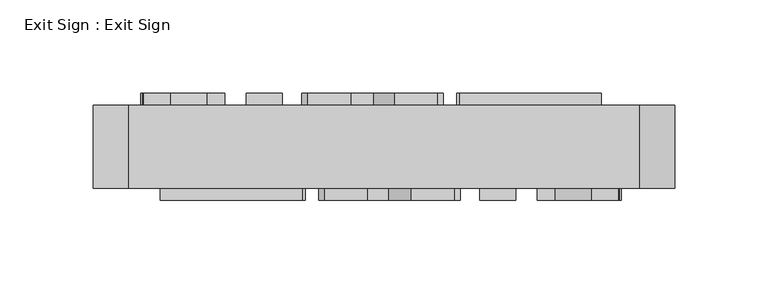
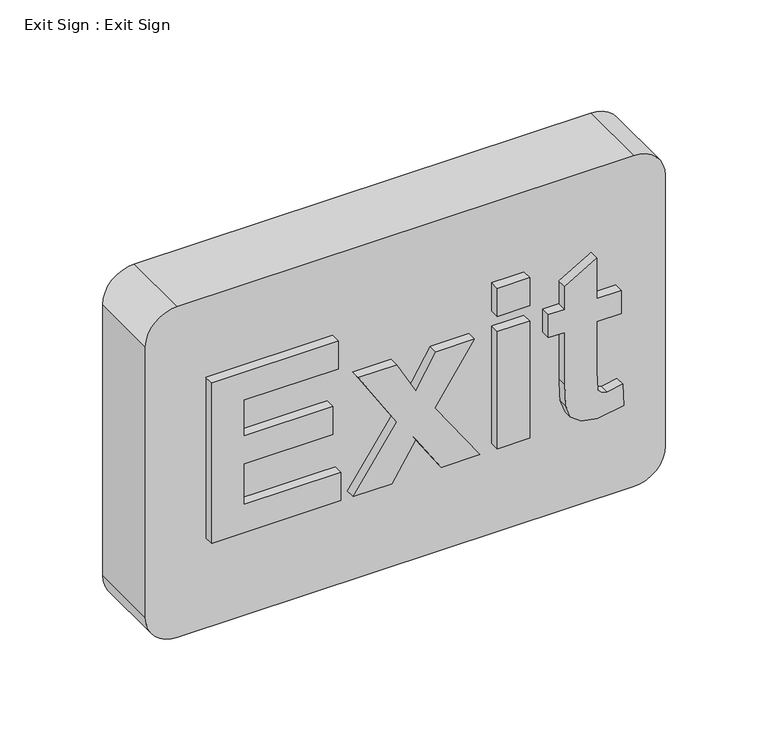
"""IFC4 building model written with IfcOpenShell, lengths in millimetres: proxy geometry, Exit Sign : Exit Sign."""

from ifc_helpers import new_model, si_unit, point, frame, frame_2d, origin, place, context, project, spatial, polyline, circle_curve, trimmed, segment, composite_curve, outline, extrude, source, transform, mapped, element, save


def exit_sign_exit_sign_daf696ad(model_context):
    return source(origin(), model_context, "Body", "SweptSolid", [
        extrude(outline(composite_curve([segment(polyline([(2438.4, 136.525), (2438.4, -136.525)]), True, "CONTINUOUS"), segment(trimmed(circle_curve(frame_2d((2419.35, -136.525)), 19.05), [point((2438.4, -136.525))], [point((2419.35, -155.575))], False, "CARTESIAN"), True, "CONTINUOUS"), segment(polyline([(2419.35, -155.575), (2247.9, -155.575)]), True, "CONTINUOUS"), segment(trimmed(circle_curve(frame_2d((2247.9, -136.525)), 19.05), [point((2247.9, -155.575))], [point((2228.85, -136.525))], False, "CARTESIAN"), True, "CONTINUOUS"), segment(polyline([(2228.85, -136.525), (2228.85, 136.525)]), True, "CONTINUOUS"), segment(trimmed(circle_curve(frame_2d((2247.9, 136.525)), 19.05), [point((2228.85, 136.525))], [point((2247.9, 155.575))], False, "CARTESIAN"), True, "CONTINUOUS"), segment(polyline([(2247.9, 155.575), (2419.35, 155.575)]), True, "CONTINUOUS"), segment(trimmed(circle_curve(frame_2d((2419.35, 136.525)), 19.05), [point((2419.35, 155.575))], [point((2438.4, 136.525))], False, "CARTESIAN"), True, "CONTINUOUS")], self_intersect=False)), frame((0.0, -34.925, 0.0), z_axis=(0.0, 1.0, 0.0), x_axis=(0.0, 0.0, 1.0)), (0.0, 0.0, 1.0), 44.45),
        extrude(outline(polyline([(2286.4280581, -119.6667099), (2286.4280581, -42.2571861), (2304.1677406, -42.2571861), (2304.1677406, -100.314329), (2329.9709152, -100.314329), (2329.9709152, -47.0952813), (2347.7105977, -47.0952813), (2347.7105977, -100.314329), (2370.2883755, -100.314329), (2370.2883755, -43.8698845), (2388.0280581, -43.8698845), (2388.0280581, -119.6667099), (2286.4280581, -119.6667099)])), frame((0.0, -41.275, 0.0), z_axis=(0.0, 1.0, 0.0), x_axis=(0.0, 0.0, 1.0)), (0.0, 0.0, 1.0), 6.35),
        extrude(outline(polyline([(2286.4280581, -35.0000432), (2286.4280581, -11.9938925), (2309.4090104, 2.4195996), (2286.4280581, 17.7906314), (2286.4280581, 40.7967822), (2325.4855977, 13.9100758), (2360.612185, 37.5713853), (2360.612185, 14.5652345), (2340.2266692, 2.4195996), (2360.612185, -8.7684956), (2360.612185, -31.7746464), (2324.6288517, -8.793694), (2286.4280581, -35.0000432)])), frame((0.0, -41.275, 0.0), z_axis=(0.0, 1.0, 0.0), x_axis=(0.0, 0.0, 1.0)), (0.0, 0.0, 1.0), 6.35),
        extrude(outline(polyline([(70.6317028, -41.275), (51.2793218, -41.275), (51.2793218, -34.925), (70.6317028, -34.925), (70.6317028, -41.275)])), frame((0.0, 0.0, 2370.2883755), z_axis=(0.0, 0.0, 1.0), x_axis=(1.0, 0.0, 0.0)), (0.0, 0.0, 1.0), 17.7396825),
        extrude(outline(polyline([(70.6317028, -41.275), (51.2793218, -41.275), (51.2793218, -34.925), (70.6317028, -34.925), (70.6317028, -41.275)])), frame((0.0, 0.0, 2286.4280581), z_axis=(0.0, 0.0, 1.0), x_axis=(1.0, 0.0, 0.0)), (0.0, 0.0, 1.0), 74.184127),
        extrude(outline(polyline([(2360.612185, 125.4634488), (2360.612185, 110.9491631), (2386.4153597, 110.9491631), (2375.1264708, 91.5967822), (2360.612185, 91.5967822), (2360.612185, 81.9205917), (2346.0978993, 81.9205917), (2346.0978993, 91.5967822), (2313.1887723, 91.5967822), (2299.1028597, 92.2267425), (2291.3165501, 95.0615639), (2286.6296454, 101.4493615), (2284.8153597, 111.2263456), (2287.4359946, 127.0761472), (2301.1943279, 126.269798), (2299.3296454, 117.1983695), (2300.3753795, 113.3934091), (2303.0212128, 111.3901353), (2314.2723041, 110.9491631), (2346.0978993, 110.9491631), (2346.0978993, 125.4634488), (2360.612185, 125.4634488)])), frame((0.0, -41.275, 0.0), z_axis=(0.0, 1.0, 0.0), x_axis=(0.0, 0.0, 1.0)), (0.0, 0.0, 1.0), 6.35),
        extrude(outline(polyline([(2284.0985242, 116.4382316), (2385.6985242, 116.4382316), (2385.6985242, 40.6414062), (2367.9588417, 40.6414062), (2367.9588417, 97.0858507), (2345.3810639, 97.0858507), (2345.3810639, 43.866803), (2327.6413814, 43.866803), (2327.6413814, 97.0858507), (2301.8382068, 97.0858507), (2301.8382068, 39.0287078), (2284.0985242, 39.0287078), (2284.0985242, 116.4382316)])), frame((0.0, 9.525, 0.0), z_axis=(0.0, 1.0, 0.0), x_axis=(0.0, 0.0, 1.0)), (0.0, 0.0, 1.0), 6.35),
        extrude(outline(polyline([(2284.0985242, 31.7715649), (2322.2993179, 5.5652157), (2358.2826512, 28.5461681), (2358.2826512, 5.5400173), (2337.8971354, -5.6480779), (2358.2826512, -17.7937128), (2358.2826512, -40.7998636), (2323.1560639, -17.1385541), (2284.0985242, -44.0252605), (2284.0985242, -21.0191097), (2307.0794766, -5.6480779), (2284.0985242, 8.7654141), (2284.0985242, 31.7715649)])), frame((0.0, 9.525, 0.0), z_axis=(0.0, 1.0, 0.0), x_axis=(0.0, 0.0, 1.0)), (0.0, 0.0, 1.0), 6.35),
        extrude(outline(polyline([(-73.8601811, 15.875), (-54.5078001, 15.875), (-54.5078001, 9.525), (-73.8601811, 9.525), (-73.8601811, 15.875)])), frame((0.0, 0.0, 2367.9588417), z_axis=(0.0, 0.0, 1.0), x_axis=(1.0, 0.0, 0.0)), (0.0, 0.0, 1.0), 17.7396825),
        extrude(outline(polyline([(-73.8601811, 15.875), (-54.5078001, 15.875), (-54.5078001, 9.525), (-73.8601811, 9.525), (-73.8601811, 15.875)])), frame((0.0, 0.0, 2284.0985242), z_axis=(0.0, 0.0, 1.0), x_axis=(1.0, 0.0, 0.0)), (0.0, 0.0, 1.0), 74.184127),
        extrude(outline(polyline([(2358.2826512, -128.6919271), (2343.7683655, -128.6919271), (2343.7683655, -114.1776414), (2311.9427703, -114.1776414), (2300.691679, -114.6186136), (2298.0458457, -116.6218874), (2297.0001115, -120.4268478), (2298.8647941, -129.4982763), (2285.1064607, -130.3046255), (2282.4858258, -114.4548239), (2284.3001115, -104.6778398), (2288.9870163, -98.2900422), (2296.7733258, -95.4552208), (2310.8592385, -94.8252605), (2343.7683655, -94.8252605), (2343.7683655, -85.14907), (2358.2826512, -85.14907), (2358.2826512, -94.8252605), (2372.7969369, -94.8252605), (2384.0858258, -114.1776414), (2358.2826512, -114.1776414), (2358.2826512, -128.6919271)])), frame((0.0, 9.525, 0.0), z_axis=(0.0, 1.0, 0.0), x_axis=(0.0, 0.0, 1.0)), (0.0, 0.0, 1.0), 6.35),
    ])


if __name__ == "__main__":
    model = new_model("IFC4")
    model_context = context("Model", 3, world=origin())
    ifc_project = project(units=[si_unit("LENGTHUNIT", "METRE", prefix="MILLI")], contexts=[model_context])
    site = spatial("IfcSite", under=ifc_project)
    building = spatial("IfcBuilding", under=site)
    placement = place(None, origin())
    exit_sign_exit_sign_shape = exit_sign_exit_sign_daf696ad(model_context)
    element("IfcBuildingElementProxy", 1, Name="Exit Sign : Exit Sign", ObjectType="Exit Sign : Exit Sign", at=placement, inside=building, context=model_context, shape_type="MappedRepresentation", body=[
        mapped(exit_sign_exit_sign_shape, transform((0.0, 0.0, 0.0), x_axis=(1.0, 0.0, 0.0), y_axis=(0.0, 1.0, 0.0), z_axis=(0.0, 0.0, 1.0))),
    ])
    save(model, "model.ifc")

# Revit data of these elements
# Type "Exit Sign : Exit Sign"
#   Assembly Code = "D5090200"
#   Default Elevation = 0
# Element 1 (IfcBuildingElementProxy, "Exit Sign : Exit Sign")
#   Materials on its faces: "Red Lettering", "Steel, Paint Finish, Ivory, Glossy"
# Materials
#   "Red Lettering": class "Miscellaneous", colour RGB 200 0 0, transparency 0
#   "Steel, Paint Finish, Ivory, Glossy": class "Metal", colour RGB 247 247 239, transparency 0, Description = "Steel, paint finish, ivory, glossy", Cost = 0
